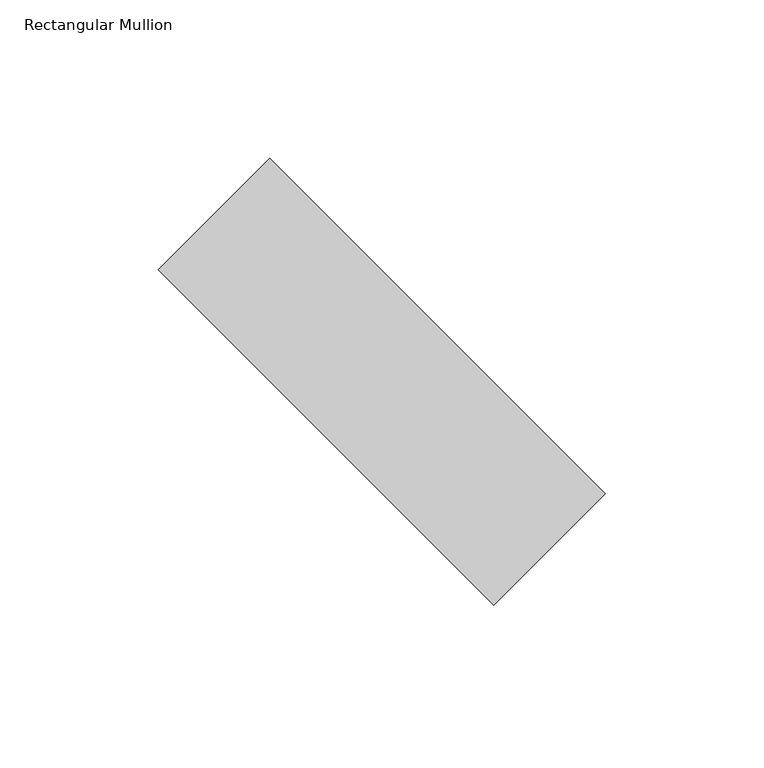
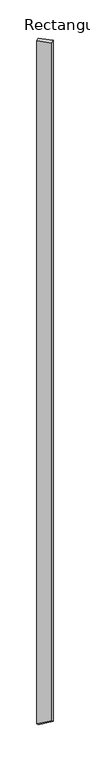
"""IFC4 building model written with IfcOpenShell, lengths in millimetres: member geometry, Rectangular Mullion : tilted mullions."""

from ifc_helpers import new_model, si_unit, origin, place, context, project, spatial, faceted_brep, source, transform, mapped, element, save


def rectangular_mullion_56583e28(model_context):
    return source(origin(), model_context, "Body", "Brep", [
        faceted_brep([(-35.3553391, 70.7106781, 0.0), (-70.7106781, 35.3553391, 0.0), (35.3553391, -70.7106781, 0.0), (70.7106781, -35.3553391, 0.0), (-35.3553391, 70.7106781, -8054.6449262), (-70.7106781, 35.3553391, -8009.5889489), (35.3553391, -70.7106781, -7944.553342), (70.7106781, -35.3553391, -7989.6093193)], [[[0, 1, 2, 3]], [[1, 0, 4, 5]], [[2, 1, 5, 6]], [[3, 2, 6, 7]], [[0, 3, 7, 4]], [[4, 7, 6, 5]]]),
    ])


if __name__ == "__main__":
    model = new_model("IFC4")
    model_context = context("Model", 3, world=origin())
    ifc_project = project(units=[si_unit("LENGTHUNIT", "METRE", prefix="MILLI")], contexts=[model_context])
    site = spatial("IfcSite", under=ifc_project)
    building = spatial("IfcBuilding", under=site)
    placement = place(None, origin())
    rectangular_mullion_shape = rectangular_mullion_56583e28(model_context)
    element("IfcMember", 1, ObjectType="Rectangular Mullion : tilted mullions", at=placement, inside=building, context=model_context, shape_type="MappedRepresentation", body=[
        mapped(rectangular_mullion_shape, transform((0.0, 0.0, 0.0), x_axis=(1.0, 0.0, 0.0), y_axis=(0.0, 1.0, 0.0), z_axis=(0.0, 0.0, 1.0))),
    ])
    save(model, "model.ifc")

# Revit data of these elements
# Type "Rectangular Mullion : tilted mullions"
#   built-in parameter 1007304 = 0.492126 (stored number, unit not read)
#   built-in parameter 1007301 = 0.082021 (stored number, unit not read)
#   built-in parameter 1007300 = 0.082021 (stored number, unit not read)
# Element 1 (IfcMember, "Rectangular Mullion : tilted mullions")
#   Materials on its faces: "Aluminum"
# Materials
#   "Aluminum": class "Metal", colour RGB 244 244 244, transparency 0, Description = "Aluminum 6061", Cost = 0
